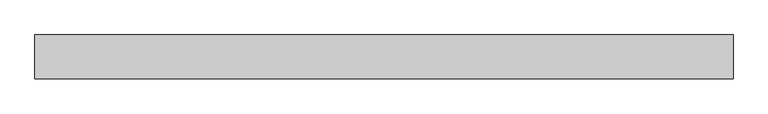
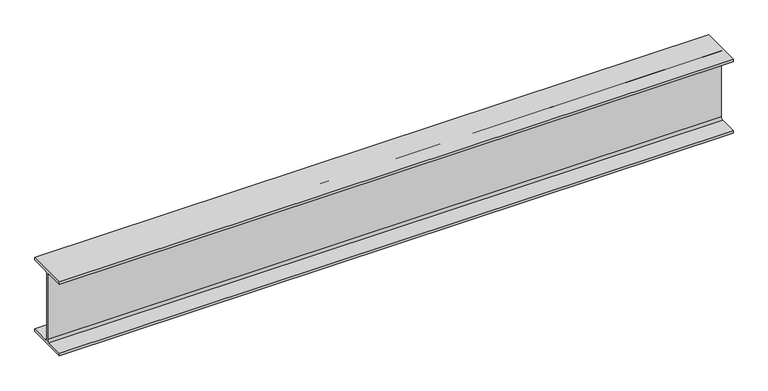
"""IFC4 building model written with IfcOpenShell, lengths in millimetres: beam geometry, Steel Beam_H-KSD3502 : H_SB_ASB_H-194x150x6x9."""

from ifc_helpers import new_model, si_unit, point, frame, frame_2d, origin, place, context, project, spatial, polyline, circle_curve, trimmed, segment, composite_curve, outline, extrude, source, transform, mapped, element, save


def beam_e9c9c49d(model_context):
    return source(origin(), model_context, "Body", "SweptSolid", [
        extrude(outline(composite_curve([segment(polyline([(82.5, -141.5), (82.5, -151.7), (-82.5, -151.7), (-82.5, -141.5), (-11.9, -141.5)]), True, "CONTINUOUS"), segment(trimmed(circle_curve(frame_2d((-11.9, -132.6)), 8.9), [point((-11.9, -141.5))], [point((-3.0, -132.6))], True, "CARTESIAN"), True, "CONTINUOUS"), segment(polyline([(-3.0, -132.6), (-3.0, 132.6)]), True, "CONTINUOUS"), segment(trimmed(circle_curve(frame_2d((-11.9, 132.6)), 8.9), [point((-3.0, 132.6))], [point((-11.9, 141.5))], True, "CARTESIAN"), True, "CONTINUOUS"), segment(polyline([(-11.9, 141.5), (-82.5, 141.5), (-82.5, 151.7), (82.5, 151.7), (82.5, 141.5), (11.9, 141.5)]), True, "CONTINUOUS"), segment(trimmed(circle_curve(frame_2d((11.9, 132.6)), 8.9), [point((11.9, 141.5))], [point((3.0, 132.6))], True, "CARTESIAN"), True, "CONTINUOUS"), segment(polyline([(3.0, 132.6), (3.0, -132.6)]), True, "CONTINUOUS"), segment(trimmed(circle_curve(frame_2d((11.9, -132.6)), 8.9), [point((3.0, -132.6))], [point((11.9, -141.5))], True, "CARTESIAN"), True, "CONTINUOUS"), segment(polyline([(11.9, -141.5), (82.5, -141.5)]), True, "CONTINUOUS")], self_intersect=False)), frame((-1068.0314701, 0.0, 0.0), z_axis=(1.0, 0.0, 0.0), x_axis=(0.0, 1.0, 0.0)), (0.0, 0.0, 1.0), 2617.0588612),
    ])


if __name__ == "__main__":
    model = new_model("IFC4")
    model_context = context("Model", 3, world=origin())
    ifc_project = project(units=[si_unit("LENGTHUNIT", "METRE", prefix="MILLI")], contexts=[model_context])
    site = spatial("IfcSite", under=ifc_project)
    building = spatial("IfcBuilding", under=site)
    placement = place(None, origin())
    beam_shape = beam_e9c9c49d(model_context)
    element("IfcBeam", 1, ObjectType="Steel Beam_H-KSD3502 : H_SB_ASB_H-194x150x6x9", at=placement, inside=building, context=model_context, shape_type="MappedRepresentation", body=[
        mapped(beam_shape, transform((0.0, 0.0, 0.0), x_axis=(1.0, 0.0, 0.0), y_axis=(0.0, 1.0, 0.0), z_axis=(0.0, 0.0, 1.0))),
    ])
    save(model, "model.ifc")

# Revit data of these elements
# Type "Steel Beam_H-KSD3502 : H_SB_ASB_H-194x150x6x9"
#   Width = 15.0 cm
#   Web Thickness = 0.6 cm
#   Web Fillet = 1.3 cm
#   Warping Constant = 43316.0 cm⁶
#   Torsional Moment of Inertia = 8.622 cm⁴
#   Torsional Modulus = 1.0 cm³
#   Section Area = 39.01 cm²
#   Plastic Modulus weak axis = 104.0 cm³
#   Plastic Modulus strong axis = 309.0 cm³
#   Perimeter = 0.95 m²/m
#   Nominal Weight = 30.60 kgf/m
#   Moment of Inertia weak axis = 507.00 cm⁴
#   Moment of Inertia strong axis = 2690.00 cm⁴
#   Height = 19.4 cm
#   Flange Thickness = 0.9 cm
#   Elastic Modulus weak axis = 67.6 cm³
#   Elastic Modulus strong axis = 277.0 cm³
#   Centroid Vertical = 9.7 cm
#   Centroid Horizontal = 7.5 cm
#   Length [instance default] = 1.5240 m
#   Structural Material [instance default] = Steel, 45-345
#   Assembly Code = ""
# Element 1 (IfcBeam, "Steel Beam_H-KSD3502 : H_SB_ASB_H-194x150x6x9")
#   Structural Material = none
# Materials
#   "Steel, 45-345": class "Metal", colour RGB 189 187 185, transparency 0, Description = "Steel 345 MPa", Cost = 0
